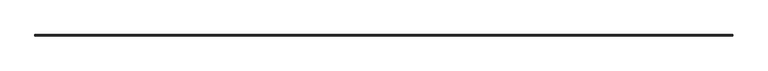
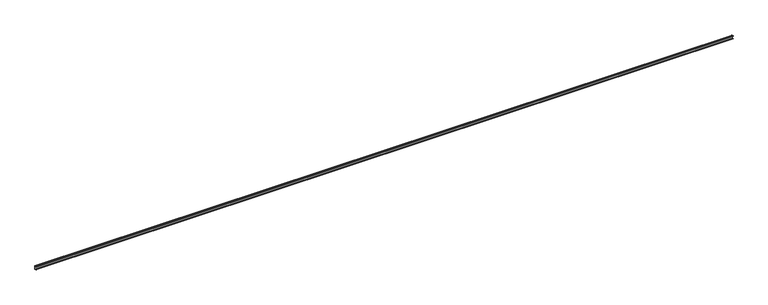
"""IFC4 building model written with IfcOpenShell, lengths in millimetres: beam geometry, 0912_Steel Framing_LC_KDS3530 : H_SB_AR_B03_LC-200x75x25x3.2."""

from ifc_helpers import new_model, si_unit, point, frame, frame_2d, origin, place, context, project, spatial, polyline, circle_curve, trimmed, segment, composite_curve, outline, extrude, source, transform, mapped, element, save


def beam_a0262063(model_context):
    return source(origin(), model_context, "Body", "SweptSolid", [
        extrude(outline(composite_curve([segment(polyline([(18.6, 87.5), (18.6, -87.5)]), True, "CONTINUOUS"), segment(trimmed(circle_curve(frame_2d((6.1, -87.5)), 12.5), [point((18.6, -87.5))], [point((6.1, -100.0))], False, "CARTESIAN"), True, "CONTINUOUS"), segment(polyline([(6.1, -100.0), (-43.9, -100.0)]), True, "CONTINUOUS"), segment(trimmed(circle_curve(frame_2d((-43.9, -87.5)), 12.5), [point((-43.9, -100.0))], [point((-56.4, -87.5))], False, "CARTESIAN"), True, "CONTINUOUS"), segment(polyline([(-56.4, -87.5), (-56.4, -75.0), (-51.9, -75.0), (-51.9, -87.5)]), True, "CONTINUOUS"), segment(trimmed(circle_curve(frame_2d((-43.9, -87.5)), 8.0), [point((-51.9, -87.5))], [point((-43.9, -95.5))], True, "CARTESIAN"), True, "CONTINUOUS"), segment(polyline([(-43.9, -95.5), (6.1, -95.5)]), True, "CONTINUOUS"), segment(trimmed(circle_curve(frame_2d((6.1, -87.5)), 8.0), [point((6.1, -95.5))], [point((14.1, -87.5))], True, "CARTESIAN"), True, "CONTINUOUS"), segment(polyline([(14.1, -87.5), (14.1, 87.5)]), True, "CONTINUOUS"), segment(trimmed(circle_curve(frame_2d((6.1, 87.5)), 8.0), [point((14.1, 87.5))], [point((6.1, 95.5))], True, "CARTESIAN"), True, "CONTINUOUS"), segment(polyline([(6.1, 95.5), (-41.1, 95.5)]), True, "CONTINUOUS"), segment(trimmed(circle_curve(frame_2d((-41.1, 87.5)), 8.0), [point((-41.1, 95.5))], [point((-49.1, 87.5))], True, "CARTESIAN"), True, "CONTINUOUS"), segment(polyline([(-49.1, 87.5), (-49.1, 75.0), (-53.6, 75.0), (-53.6, 87.5)]), True, "CONTINUOUS"), segment(trimmed(circle_curve(frame_2d((-41.1, 87.5)), 12.5), [point((-53.6, 87.5))], [point((-41.1, 100.0))], False, "CARTESIAN"), True, "CONTINUOUS"), segment(polyline([(-41.1, 100.0), (6.1, 100.0)]), True, "CONTINUOUS"), segment(trimmed(circle_curve(frame_2d((6.1, 87.5)), 12.5), [point((6.1, 100.0))], [point((18.6, 87.5))], False, "CARTESIAN"), True, "CONTINUOUS")], self_intersect=False)), frame((-19650.0, 0.0, 0.0), z_axis=(1.0, 0.0, 0.0), x_axis=(0.0, 1.0, 0.0)), (0.0, 0.0, 1.0), 39300.0),
    ])


if __name__ == "__main__":
    model = new_model("IFC4")
    model_context = context("Model", 3, world=origin())
    ifc_project = project(units=[si_unit("LENGTHUNIT", "METRE", prefix="MILLI")], contexts=[model_context])
    site = spatial("IfcSite", under=ifc_project)
    building = spatial("IfcBuilding", under=site)
    placement = place(None, origin())
    beam_shape = beam_a0262063(model_context)
    element("IfcBeam", 1, ObjectType="0912_Steel Framing_LC_KDS3530 : H_SB_AR_B03_LC-200x75x25x3.2", at=placement, inside=building, context=model_context, shape_type="MappedRepresentation", body=[
        mapped(beam_shape, transform((0.0, 0.0, 0.0), x_axis=(1.0, 0.0, 0.0), y_axis=(0.0, 1.0, 0.0), z_axis=(0.0, 0.0, 1.0))),
    ])
    save(model, "model.ifc")

# Revit data of these elements
# Type "0912_Steel Framing_LC_KDS3530 : H_SB_AR_B03_LC-200x75x25x3.2"
#   r = 8 mm
#   d = 25 mm
#   R = 11.2 mm
#   Perimeter = 0.78 m²/m
#   Nominal Weight = 14.00 kgf/m
#   Length [instance default] = 1000 mm
#   B = 75 mm
#   H = 200 mm
#   tw = 3.2 mm
#   x = 18.6 mm
#   A = 1.00 m²
#   Structural Material [instance default] = Steel, 45-345
#   Assembly Code = ""
# Element 1 (IfcBeam, "0912_Steel Framing_LC_KDS3530 : H_SB_AR_B03_LC-200x75x25x3.2")
#   Structural Material = Steel ASTM A36
#   Materials on its faces: "Steel ASTM A36"
# Materials
#   "Steel, 45-345": class "Metal", colour RGB 189 187 185, transparency 0, Description = "Steel 345 MPa", Cost = 0
#   "Steel ASTM A36": class "Metal", colour RGB 199 199 199, transparency 0, Description = "Structural steel, ASTM A36 Grade B, mill finish", Cost = 0
